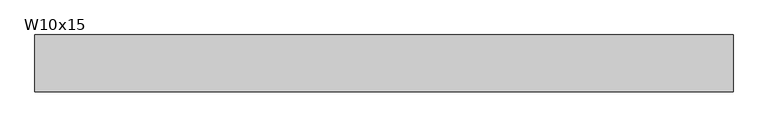
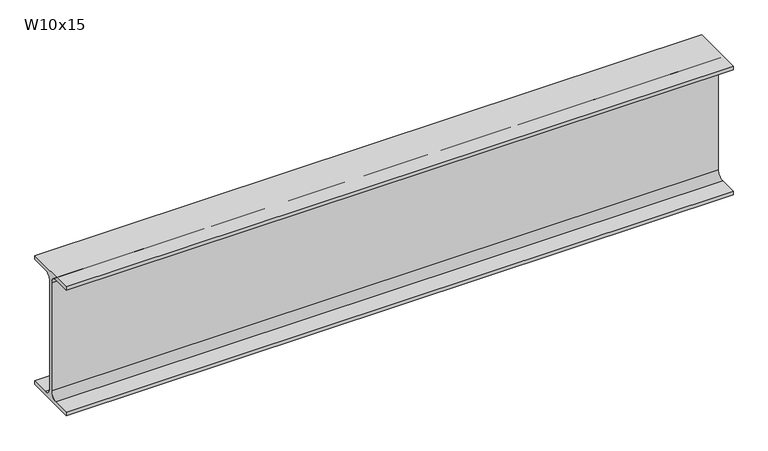
"""IFC4 building model written with IfcOpenShell, lengths in millimetres: beam geometry, RME W-Wide Flange : W10x15."""

from ifc_helpers import new_model, si_unit, point, frame, frame_2d, origin, place, context, project, spatial, polyline, circle_curve, trimmed, segment, composite_curve, outline, extrude, source, transform, mapped, element, save


def w10x15_6b6119be(model_context):
    return source(origin(), model_context, "Body", "SweptSolid", [
        extrude(outline(composite_curve([segment(polyline([(50.8, -120.142), (50.8, -127.0), (-50.8, -127.0), (-50.8, -120.142), (-16.7005, -120.142)]), True, "CONTINUOUS"), segment(trimmed(circle_curve(frame_2d((-16.7005, -106.3625)), 13.7795), [point((-16.7005, -120.142))], [point((-2.921, -106.3625))], True, "CARTESIAN"), True, "CONTINUOUS"), segment(polyline([(-2.921, -106.3625), (-2.921, 106.3625)]), True, "CONTINUOUS"), segment(trimmed(circle_curve(frame_2d((-16.7005, 106.3625)), 13.7795), [point((-2.921, 106.3625))], [point((-16.7005, 120.142))], True, "CARTESIAN"), True, "CONTINUOUS"), segment(polyline([(-16.7005, 120.142), (-50.8, 120.142), (-50.8, 127.0), (50.8, 127.0), (50.8, 120.142), (16.7005, 120.142)]), True, "CONTINUOUS"), segment(trimmed(circle_curve(frame_2d((16.7005, 106.3625)), 13.7795), [point((16.7005, 120.142))], [point((2.921, 106.3625))], True, "CARTESIAN"), True, "CONTINUOUS"), segment(polyline([(2.921, 106.3625), (2.921, -106.3625)]), True, "CONTINUOUS"), segment(trimmed(circle_curve(frame_2d((16.7005, -106.3625)), 13.7795), [point((2.921, -106.3625))], [point((16.7005, -120.142))], True, "CARTESIAN"), True, "CONTINUOUS"), segment(polyline([(16.7005, -120.142), (50.8, -120.142)]), True, "CONTINUOUS")], self_intersect=False)), frame((-583.819, 0.0, 0.0), z_axis=(1.0, 0.0, 0.0), x_axis=(0.0, 1.0, 0.0)), (0.0, 0.0, 1.0), 1244.219),
    ])


if __name__ == "__main__":
    model = new_model("IFC4")
    model_context = context("Model", 3, world=origin())
    ifc_project = project(units=[si_unit("LENGTHUNIT", "METRE", prefix="MILLI")], contexts=[model_context])
    site = spatial("IfcSite", under=ifc_project)
    building = spatial("IfcBuilding", under=site)
    placement = place(None, origin())
    w10x15_shape = w10x15_6b6119be(model_context)
    element("IfcBeam", 1, ObjectType="RME W-Wide Flange : W10x15", at=placement, inside=building, context=model_context, shape_type="MappedRepresentation", body=[
        mapped(w10x15_shape, transform((0.0, 0.0, 0.0), x_axis=(1.0, 0.0, 0.0), y_axis=(0.0, 1.0, 0.0), z_axis=(0.0, 0.0, 1.0))),
    ])
    save(model, "model.ifc")

# Revit data of these elements
# Type "RME W-Wide Flange : W10x15"
#   WELD P [instance default] = ""
#   WELD LE [instance default] = ""
#   WELD D [instance default] = ""
#   TOP SECTION SIZE [instance default] = ""
#   TOP SECTION LENGTH [instance default] = ""
#   REMARKS [instance default] = ""
#   REINF TYPE [instance default] = ""
#   Nominal Size = "W24"
#   End Bearing Capacity [instance default] = ""
#   BOT SECTION SIZE [instance default] = ""
#   BOT SECTION LENGTH [instance default] = ""
#   Assembly Code = "B10"
#   W = 15
#   Start Extension Calculation [instance default] = 10' - 0"
#   Start Extension [instance default] = -0' - 0 1/2"
#   End Extension Calculation [instance default] = 10' - 0"
#   End Extension [instance default] = -0' - 0 1/2"
#   Length [instance default] = 5' - 0"
#   bf = 0' - 4"
#   d = 0' - 10"
#   k = 0' - 0 13/16"
#   k2 = 0' - 0.5425"
#   tf = 0' - 0.27"
#   tw = 0' - 0.23"
#   A = 0.030625 SF
#   Structural Material [instance default] = Metal - Steel - ASTM A992
# Element 1 (IfcBeam, "RME W-Wide Flange : W10x15")
#   Length = 4' - 4"
#   Materials on its faces: "Metal - Steel - ASTM A992"
# Materials
#   "Metal - Steel - ASTM A992": class "Metal", colour RGB 255 128 0, transparency 0
